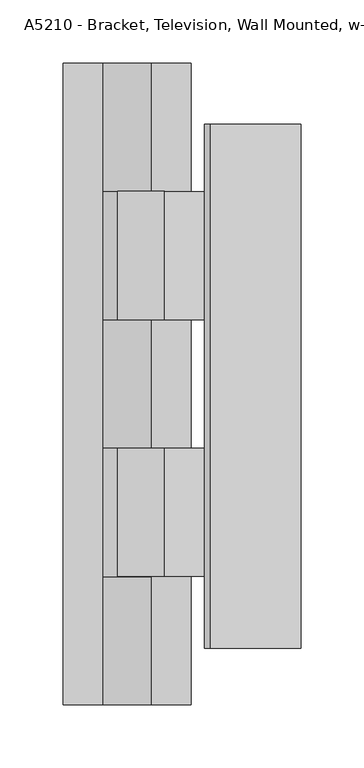
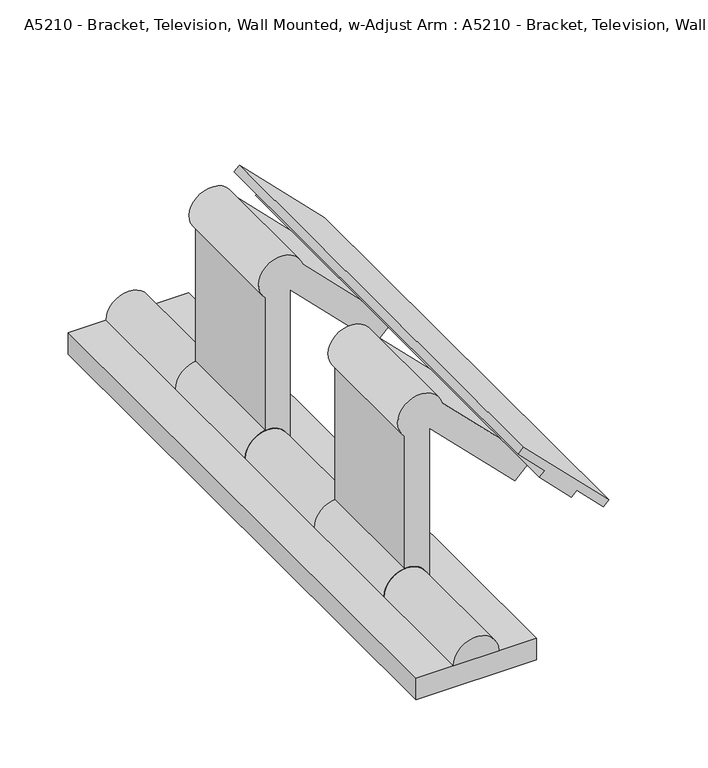
"""IFC4 building model written with IfcOpenShell, lengths in millimetres: proxy geometry, A5210 - Bracket, Television, Wall Mounted, w-Adjust Arm : A5210 - Bracket, Television, Wall Mounted, w-Adjust Arm."""

from ifc_helpers import new_model, si_unit, point, frame, frame_2d, origin, origin_with_axes, place, context, project, spatial, polyline, circle_curve, trimmed, segment, composite_curve, outline, extrude, source, transform, mapped, element, save


def a5210_bracket_television_wall_mounted_w_adjust_arm_a5210_bc629ad1(model_context):
    return source(origin(), model_context, "Body", "SweptSolid", [
        extrude(outline(polyline([(156.8608033, 65.7508765), (152.3706752, 61.2607484), (129.9200349, 83.7113887), (125.4299069, 79.2212606), (98.4891385, 106.162029), (102.9792666, 110.6521571), (80.5286263, 133.1027974), (85.0187543, 137.5929254), (156.8608033, 65.7508765)])), frame((0.0, 44.6660281, 0.0), z_axis=(0.0, 1.0, 0.0), x_axis=(0.0, 0.0, 1.0)), (0.0, 0.0, 1.0), 415.0622238),
        extrude(outline(composite_curve([segment(polyline([(155.914578, 19.05), (83.6458437, 91.3187342), (98.4891385, 106.162029), (174.8504925, 29.800675)]), True, "CONTINUOUS"), segment(trimmed(circle_curve(frame_2d((169.6547742, 11.4729089)), 19.05), [point((174.8504925, 29.800675))], [point((156.1287345, -1.9415888))], False, "CARTESIAN"), True, "CONTINUOUS"), segment(polyline([(156.1287345, -1.9415888), (38.3178779, -1.9415888)]), True, "CONTINUOUS"), segment(trimmed(circle_curve(frame_2d((19.3787695, 0.1108917)), 19.05), [point((38.3178779, -1.9415888))], [point((21.43125, 19.05))], True, "CARTESIAN"), True, "CONTINUOUS"), segment(polyline([(21.43125, 19.05), (155.914578, 19.05)]), True, "CONTINUOUS")], self_intersect=False)), frame((0.0, 101.6, 0.0), z_axis=(0.0, 1.0, 0.0), x_axis=(0.0, 0.0, 1.0)), (0.0, 0.0, 1.0), 101.6),
        extrude(outline(composite_curve([segment(polyline([(155.914578, 19.05), (83.6458437, 91.3187342), (98.4891385, 106.162029), (174.8504925, 29.800675)]), True, "CONTINUOUS"), segment(trimmed(circle_curve(frame_2d((169.6547742, 11.4729089)), 19.05), [point((174.8504925, 29.800675))], [point((156.1287345, -1.9415888))], False, "CARTESIAN"), True, "CONTINUOUS"), segment(polyline([(156.1287345, -1.9415888), (38.3178779, -1.9415888)]), True, "CONTINUOUS"), segment(trimmed(circle_curve(frame_2d((19.3787695, 0.1108917)), 19.05), [point((38.3178779, -1.9415888))], [point((21.43125, 19.05))], True, "CARTESIAN"), True, "CONTINUOUS"), segment(polyline([(21.43125, 19.05), (155.914578, 19.05)]), True, "CONTINUOUS")], self_intersect=False)), frame((0.0, 304.8, 0.0), z_axis=(0.0, 1.0, 0.0), x_axis=(0.0, 0.0, 1.0)), (0.0, 0.0, 1.0), 101.6),
        extrude(outline(composite_curve([segment(trimmed(circle_curve(frame_2d((19.05, 0.0)), 19.05), [point((19.05, 19.05))], [point((19.05, -19.05))], False, "CARTESIAN"), True, "CONTINUOUS"), segment(polyline([(19.05, -19.05), (19.05, 19.05)]), True, "CONTINUOUS")], self_intersect=False)), frame((0.0, 101.6, 0.0), z_axis=(0.0, 1.0, 0.0), x_axis=(0.0, 0.0, 1.0)), (0.0, 0.0, 1.0), 101.6),
        extrude(outline(composite_curve([segment(trimmed(circle_curve(frame_2d((19.05, 0.0)), 19.05), [point((19.05, 19.05))], [point((19.05, -19.05))], False, "CARTESIAN"), True, "CONTINUOUS"), segment(polyline([(19.05, -19.05), (19.05, 19.05)]), True, "CONTINUOUS")], self_intersect=False)), frame((0.0, 304.8, 0.0), z_axis=(0.0, 1.0, 0.0), x_axis=(0.0, 0.0, 1.0)), (0.0, 0.0, 1.0), 101.6),
        extrude(outline(composite_curve([segment(polyline([(19.05, -19.05), (19.05, 19.05)]), True, "CONTINUOUS"), segment(trimmed(circle_curve(frame_2d((19.05, 0.0)), 19.05), [point((19.05, 19.05))], [point((19.05, -19.05))], False, "CARTESIAN"), True, "CONTINUOUS")], self_intersect=False)), frame((0.0, 0.0, 0.0), z_axis=(0.0, 1.0, 0.0), x_axis=(0.0, 0.0, 1.0)), (0.0, 0.0, 1.0), 101.6),
        extrude(outline(composite_curve([segment(polyline([(19.05, -19.05), (19.05, 19.05)]), True, "CONTINUOUS"), segment(trimmed(circle_curve(frame_2d((19.05, 0.0)), 19.05), [point((19.05, 19.05))], [point((19.05, -19.05))], False, "CARTESIAN"), True, "CONTINUOUS")], self_intersect=False)), frame((0.0, 203.2, 0.0), z_axis=(0.0, 1.0, 0.0), x_axis=(0.0, 0.0, 1.0)), (0.0, 0.0, 1.0), 101.6),
        extrude(outline(composite_curve([segment(polyline([(19.05, -19.05), (19.05, 19.05)]), True, "CONTINUOUS"), segment(trimmed(circle_curve(frame_2d((19.05, 0.0)), 19.05), [point((19.05, 19.05))], [point((19.05, -19.05))], False, "CARTESIAN"), True, "CONTINUOUS")], self_intersect=False)), frame((0.0, 406.4, 0.0), z_axis=(0.0, 1.0, 0.0), x_axis=(0.0, 0.0, 1.0)), (0.0, 0.0, 1.0), 101.6),
        extrude(outline(polyline([(50.8, 0.0), (-50.8, 0.0), (-50.8, 508.0), (50.8, 508.0), (50.8, 0.0)])), origin_with_axes(), (0.0, 0.0, 1.0), 19.05),
    ])


if __name__ == "__main__":
    model = new_model("IFC4")
    model_context = context("Model", 3, world=origin())
    ifc_project = project(units=[si_unit("LENGTHUNIT", "METRE", prefix="MILLI")], contexts=[model_context])
    site = spatial("IfcSite", under=ifc_project)
    building = spatial("IfcBuilding", under=site)
    placement = place(None, origin())
    a5210_bracket_television_wall_mounted_w_adjust_arm_a5210_shape = a5210_bracket_television_wall_mounted_w_adjust_arm_a5210_bc629ad1(model_context)
    element("IfcBuildingElementProxy", 1, Name="A5210 - Bracket, Television, Wall Mounted, w-Adjust Arm : A5210 - Bracket, Television, Wall Mounted, w-Adjust Arm", ObjectType="A5210 - Bracket, Television, Wall Mounted, w-Adjust Arm : A5210 - Bracket, Television, Wall Mounted, w-Adjust Arm", at=placement, inside=building, context=model_context, shape_type="MappedRepresentation", body=[
        mapped(a5210_bracket_television_wall_mounted_w_adjust_arm_a5210_shape, transform((0.0, 0.0, 0.0), x_axis=(1.0, 0.0, 0.0), y_axis=(0.0, 1.0, 0.0), z_axis=(0.0, 0.0, 1.0))),
    ])
    save(model, "model.ifc")

# Revit data of these elements
# Type "A5210 - Bracket, Television, Wall Mounted, w-Adjust Arm : A5210 - Bracket, Television, Wall Mounted, w-Adjust Arm"
#   Watts2 = "0"
#   Watts1 = "0"
#   Unit_Issue = "EA"
#   UTIL_6_Misc = "-"
#   UTIL_5_NonMedGas = "-"
#   UTIL_4_MiscGas = "-"
#   UTIL_3_MedGas = "-"
#   UTIL_2_Elec = "-"
#   UTIL_1_WaterDrain = "-"
#   Nomenclature = "Bracket, Television, Wall Mounted, w/Adjust Arm"
#   NSN = "7730"
#   Location [instance default] = ""
#   JSN = "A5210"
#   Fund_Source_VA = "-"
#   Fund_Source_Navy = "-"
#   Fund_Source_Army = "-"
#   Fund_Source_AF = "-"
#   ELEC_Volts2 = "0"
#   ELEC_Volts1 = "0"
#   ELEC_Phase2 = "0"
#   ELEC_Phase1 = "0"
#   ELEC_HertzSwitch = "0"
#   ELEC_HertzDependent = "0"
#   ELEC_Hertz = "0"
#   ELEC_Amps2 = "0"
#   ELEC_Amps1 = "0"
#   DetailDescription = "Wall mounted television bracket with adjustable arm. Consists of movable arm with minimum 120 degree swivel. Designed for holding wall mounted, flat panel television units in patient rooms."
#   CAT_VA = "A"
#   CAT_Navy = "A"
#   CAT_IHS = "-"
#   CAT_Army = "A"
#   CAT_AF = "A"
#   BTUperhour = "0"
#   Weight_IP = 24
#   Default Elevation = 5' - 0"
#   DIM_Width_IP = 1' - 9"
#   DIM_Height_IP = 1' - 7"
#   DIM_Depth_IP = 1' - 1"
